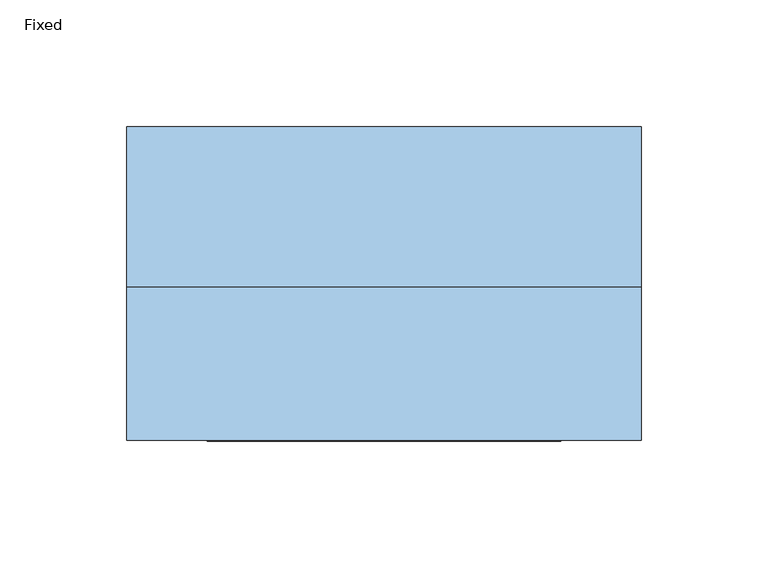
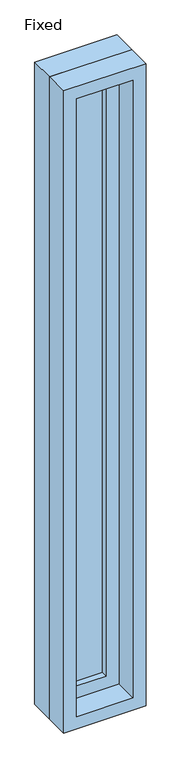
"""IFC4 building model written with IfcOpenShell, lengths in millimetres: window geometry, Fixed."""

from ifc_helpers import new_model, si_unit, frame, origin, place, context, project, spatial, polyline, outline, extrude, source, transform, mapped, element, save


def fixed_8e8cf147(model_context):
    return source(origin(), model_context, "Body", "SweptSolid", [
        extrude(outline(polyline([(0.0, 14.2875), (-76.2, 14.2875), (-76.2, 26.9875), (0.0, 26.9875), (0.0, 14.2875)])), frame((0.0, 0.0, 825.5), z_axis=(0.0, 0.0, 1.0), x_axis=(1.0, 0.0, 0.0)), (0.0, 0.0, 1.0), 1549.4),
        extrude(outline(polyline([(2419.35, -120.65), (781.05, -120.65), (781.05, 44.45), (2419.35, 44.45), (2419.35, -120.65)]), holes=[polyline([(2374.9, -76.2), (2374.9, 0.0), (825.5, 0.0), (825.5, -76.2), (2374.9, -76.2)])]), frame((0.0, -1.5875, 0.0), z_axis=(0.0, 1.0, 0.0), x_axis=(0.0, 0.0, 1.0)), (0.0, 0.0, 1.0), 44.45),
        extrude(outline(polyline([(2438.4, -139.7), (762.0, -139.7), (762.0, 63.5), (2438.4, 63.5), (2438.4, -139.7)]), holes=[polyline([(2406.65, -107.95), (2406.65, 31.75), (793.75, 31.75), (793.75, -107.95), (2406.65, -107.95)])]), frame((0.0, -61.9125, 0.0), z_axis=(0.0, 1.0, 0.0), x_axis=(0.0, 0.0, 1.0)), (0.0, 0.0, 1.0), 60.325),
        extrude(outline(polyline([(2438.4, 63.5), (2438.4, -139.7), (762.0, -139.7), (762.0, 63.5), (2438.4, 63.5)]), holes=[polyline([(2419.35, 44.45), (781.05, 44.45), (781.05, -120.65), (2419.35, -120.65), (2419.35, 44.45)])]), frame((0.0, -1.5875, 0.0), z_axis=(0.0, 1.0, 0.0), x_axis=(0.0, 0.0, 1.0)), (0.0, 0.0, 1.0), 63.5),
    ])


if __name__ == "__main__":
    model = new_model("IFC4")
    model_context = context("Model", 3, world=origin())
    ifc_project = project(units=[si_unit("LENGTHUNIT", "METRE", prefix="MILLI")], contexts=[model_context])
    site = spatial("IfcSite", under=ifc_project)
    building = spatial("IfcBuilding", under=site)
    placement = place(None, origin())
    fixed_shape = fixed_8e8cf147(model_context)
    element("IfcWindow", 1, ObjectType="Fixed : 66\" x 8\"  Screen", at=placement, inside=building, context=model_context, shape_type="MappedRepresentation", body=[
        mapped(fixed_shape, transform((0.0, 0.0, 0.0), x_axis=(1.0, 0.0, 0.0), y_axis=(0.0, 1.0, 0.0), z_axis=(0.0, 0.0, 1.0))),
    ])
    save(model, "model.ifc")

# Revit data of these elements
# Type "Fixed : 66\" x 8\"  Screen"
#   Type Mark = "71"
#   COBie.Type.CreatedBy = "doug.wood@us.ibm.com"
#   COBie.Type.CreatedOn = "2016-04-14T02:07:26"
#   COBie.Type.Name = "Windows_Fixed_66\" x 8\"  Screen_71"
#   COBie.Type.Category = "23-30 20 17 11 : Fixed Windows"
#   COBie.Type.Description = "Fixed_66\" x 8\"  Screen"
#   COBie.Type.Manufacturer = ""
#   COBie.Type.ModelNumber = ""
#   Construction Type Id = "GSP4R"
#   Assembly Code = "B2020100"
#   Analytic Construction = "1/8 in Pilkington single glazing"
#   COBie.Type.ReplacementCost = 0
#   Visual Light Transmittance = 0.9
#   Solar Heat Gain Coefficient = 0.78
#   Heat Transfer Coefficient (U) = 3.6886 W/(m²·K)
#   Height = 5' - 6"
#   Default Sill Height = 2' - 6"
#   Width = 0' - 8"
#   Window Inset = 0' - 0 3/4"
#   COBie.Type = no
#   Glass Pane Material = Screen
#   Sash Material = Sash - White
#   Wall Closure = (empty or 0)
# Element 1 (IfcWindow, "Fixed : 66\" x 8\"  Screen")
#   Materials on its faces: "Sash - White", "Screen"
# Materials
#   "Screen": class "Metal", colour RGB 120 120 120, transparency 0, Description = "Screen", Cost = 0
#   "Sash - White": class "Wood", colour RGB 255 255 255, transparency 0, Cost = 0
